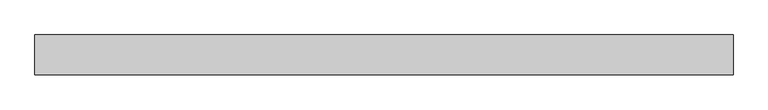
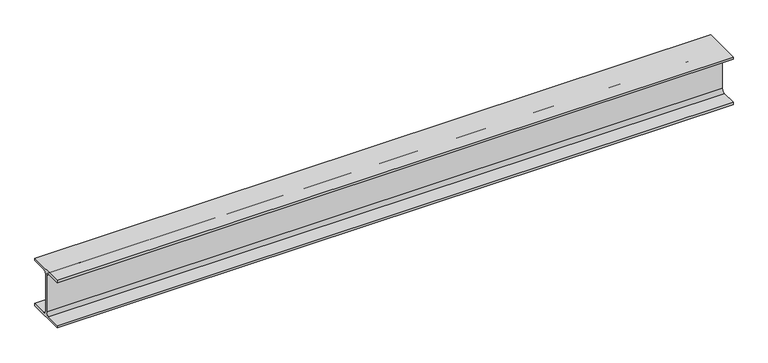
"""IFC4 building model written with IfcOpenShell, lengths in millimetres: beam geometry, 0912_Steel Framing_H-KSD3502 : H_SB_ASB_H-194x150x6x9."""

from ifc_helpers import new_model, si_unit, point, frame, frame_2d, origin, place, context, project, spatial, polyline, circle_curve, trimmed, segment, composite_curve, outline, extrude, source, transform, mapped, element, save


def beam_8b6bb364(model_context):
    return source(origin(), model_context, "Body", "SweptSolid", [
        extrude(outline(composite_curve([segment(polyline([(75.0, -88.0), (75.0, -97.0), (-75.0, -97.0), (-75.0, -88.0), (-16.0, -88.0)]), True, "CONTINUOUS"), segment(trimmed(circle_curve(frame_2d((-16.0, -75.0)), 13.0), [point((-16.0, -88.0))], [point((-3.0, -75.0))], True, "CARTESIAN"), True, "CONTINUOUS"), segment(polyline([(-3.0, -75.0), (-3.0, 75.0)]), True, "CONTINUOUS"), segment(trimmed(circle_curve(frame_2d((-16.0, 75.0)), 13.0), [point((-3.0, 75.0))], [point((-16.0, 88.0))], True, "CARTESIAN"), True, "CONTINUOUS"), segment(polyline([(-16.0, 88.0), (-75.0, 88.0), (-75.0, 97.0), (75.0, 97.0), (75.0, 88.0), (16.0, 88.0)]), True, "CONTINUOUS"), segment(trimmed(circle_curve(frame_2d((16.0, 75.0)), 13.0), [point((16.0, 88.0))], [point((3.0, 75.0))], True, "CARTESIAN"), True, "CONTINUOUS"), segment(polyline([(3.0, 75.0), (3.0, -75.0)]), True, "CONTINUOUS"), segment(trimmed(circle_curve(frame_2d((16.0, -75.0)), 13.0), [point((3.0, -75.0))], [point((16.0, -88.0))], True, "CARTESIAN"), True, "CONTINUOUS"), segment(polyline([(16.0, -88.0), (75.0, -88.0)]), True, "CONTINUOUS")], self_intersect=False)), frame((-1068.0314701, 0.0, 0.0), z_axis=(1.0, 0.0, 0.0), x_axis=(0.0, 1.0, 0.0)), (0.0, 0.0, 1.0), 2617.0588612),
    ])


if __name__ == "__main__":
    model = new_model("IFC4")
    model_context = context("Model", 3, world=origin())
    ifc_project = project(units=[si_unit("LENGTHUNIT", "METRE", prefix="MILLI")], contexts=[model_context])
    site = spatial("IfcSite", under=ifc_project)
    building = spatial("IfcBuilding", under=site)
    placement = place(None, origin())
    beam_shape = beam_8b6bb364(model_context)
    element("IfcBeam", 1, ObjectType="0912_Steel Framing_H-KSD3502 : H_SB_ASB_H-194x150x6x9", at=placement, inside=building, context=model_context, shape_type="MappedRepresentation", body=[
        mapped(beam_shape, transform((0.0, 0.0, 0.0), x_axis=(1.0, 0.0, 0.0), y_axis=(0.0, 1.0, 0.0), z_axis=(0.0, 0.0, 1.0))),
    ])
    save(model, "model.ifc")

# Revit data of these elements
# Type "0912_Steel Framing_H-KSD3502 : H_SB_ASB_H-194x150x6x9"
#   H_WM Code_1 = "S01AA002-00001 | Main Steel Structure Fabrication Work | Shelter/Building | Medium Steel - Standard (90KG/M>Weight≥30KG/M) | Material: (   )"
#   H_WM Code_2 = "S03AA028-00001 | Main Steel Structure Erection Work | Shelter/Building | Medium Steel (90KG/M>Weight≥30KG/M) | Material: (   )"
#   H_WM Code_3 = "S01AA010-00001 | Main Steel Structure Fabrication Work | Shelter/Building | Steel Painting/Coating | for Non-Fireproofed Steel Surface, Surface Preparation, Primer, Second & Final Coat | Material: (   )"
#   H_Q'ty Cal Type Tag = "SB-Q2"
#   Width = 15.0 cm
#   Web Thickness = 0.6 cm
#   Web Fillet = 1.3 cm
#   Warping Constant = 43316.0 cm⁶
#   W = 0
#   Torsional Moment of Inertia = 8.622 cm⁴
#   Section Area = 39.01 cm²
#   Plastic Modulus weak axis = 104.0 cm³
#   Plastic Modulus strong axis = 309.0 cm³
#   Perimeter = 0.95 m²/m
#   Nominal Weight = 30.60 kgf/m
#   Moment of Inertia weak axis = 507.00 cm⁴
#   Moment of Inertia strong axis = 2690.00 cm⁴
#   Height = 19.4 cm
#   Flange Thickness = 0.9 cm
#   Elastic Modulus weak axis = 67.6 cm³
#   Elastic Modulus strong axis = 277.0 cm³
#   Centroid Vertical = 9.7 cm
#   Centroid Horizontal = 7.5 cm
#   Ix = 26900000
#   Length [instance default] = 1.5240 m
#   Zx = 309000
#   b = 0.1500 m
#   h = 0.1940 m
#   r = 0.0130 m
#   s = 0.0060 m
#   t = 0.0090 m
#   A = 0.003901 m²
#   Structural Material [instance default] = Steel, 45-345
#   Assembly Code = ""
# Element 1 (IfcBeam, "0912_Steel Framing_H-KSD3502 : H_SB_ASB_H-194x150x6x9")
#   Structural Material = none
# Materials
#   "Steel, 45-345": class "Metal", colour RGB 189 187 185, transparency 0, Description = "Steel 345 MPa", Cost = 0
